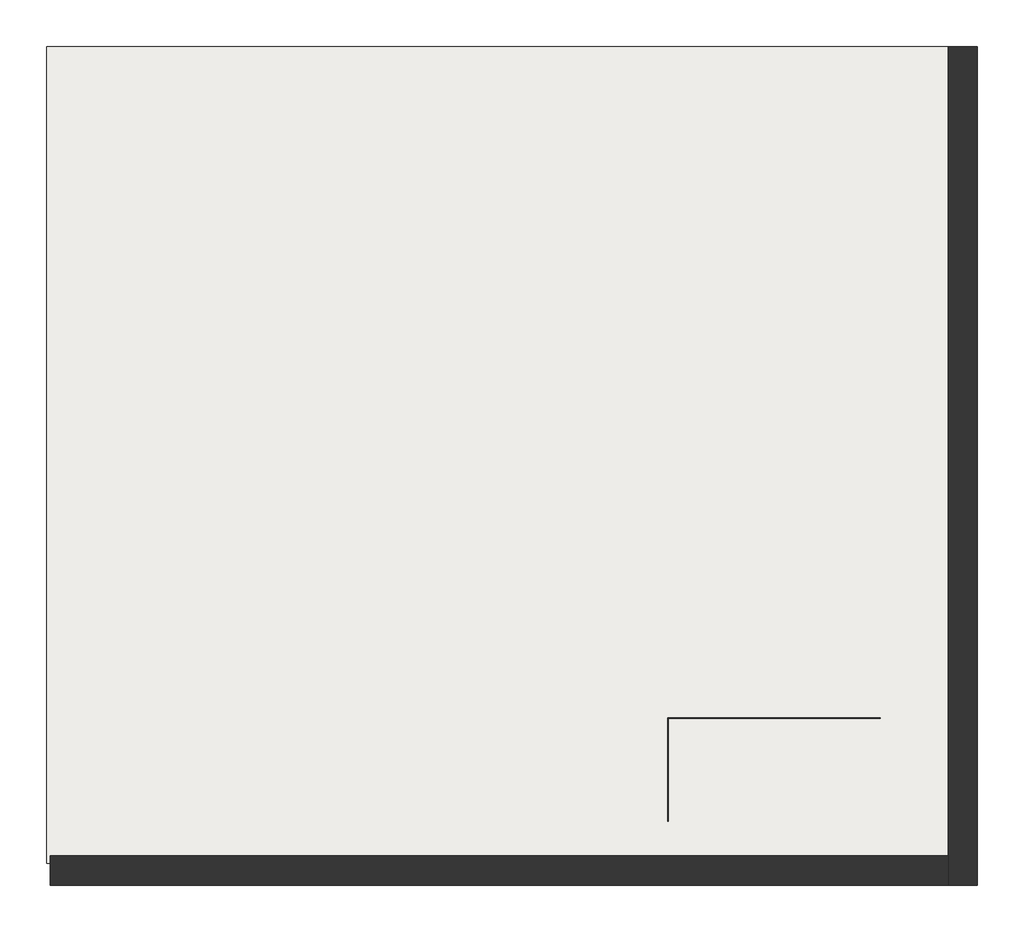
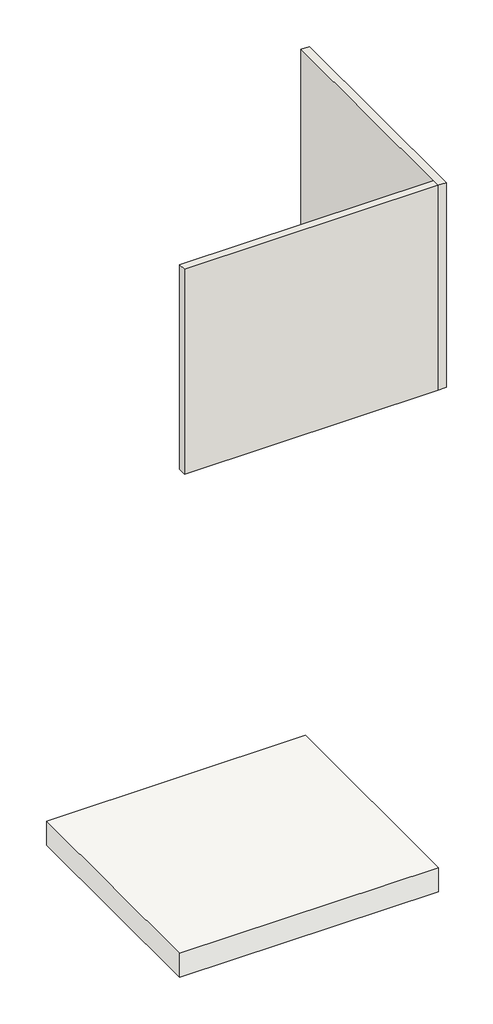
# One storey: 4 walls, 1 slab.
"""IFC4 building model written with IfcOpenShell, lengths in millimetres."""

from ifc_helpers import new_model, si_unit, frame, origin, origin_with_axes, place, context, project, spatial, polyline, outline, extrude, faceted_brep, element, save

model = new_model("IFC4")

# Units and contexts
model_context = context("Model", 3, world=origin())
ifc_project = project(units=[si_unit("LENGTHUNIT", "METRE", prefix="MILLI")], contexts=[model_context])

# Site, building, storey
site = spatial("IfcSite", under=ifc_project)
building = spatial("IfcBuilding", under=site)
storey = spatial("IfcBuildingStorey", under=building, Name="Döşeme", Elevation=0.0)

# Slab
placement = place(None, origin())
element("IfcSlab", 1, ObjectType="Generic - 12\"", at=placement, inside=storey, context=model_context, shape_type="SweptSolid", body=[
    extrude(outline(polyline([(23868.9519544, 5821.7472359), (23868.9519544, 3048.0496219), (20756.9519544, 3048.0496219), (20756.9519544, 5821.7472359), (23868.9519544, 5821.7472359)])), frame((0.0, 0.0, -6432.6532819), z_axis=(0.0, 0.0, 1.0), x_axis=(1.0, 0.0, 0.0)), (0.0, 0.0, 1.0), 304.8),
])

# Walls
element("IfcWall", 2, ObjectType="aa Marble  - 20 mm Siyah", at=placement, inside=storey, context=model_context, shape_type="Brep", body=[
    faceted_brep([(22868.9519544, 3189.0125888, 0.0), (22868.9519544, 3538.0125888, 0.0), (22868.9519544, 3540.0125888, 0.0), (22868.9519544, 3540.0125888, 390.0), (22868.9519544, 3538.0125888, 390.0), (22868.9519544, 3189.0125888, 390.0), (22866.9519544, 3189.0125888, 0.0), (22866.9519544, 3189.0125888, 390.0), (22866.9519544, 3540.0125888, 390.0), (22866.9519544, 3540.0125888, 0.0)], [[[0, 1, 2, 3, 4, 5]], [[6, 7, 8, 9]], [[3, 2, 9, 8]], [[2, 1, 0, 6, 9]], [[5, 4, 3, 8, 7]], [[0, 5, 7, 6]]]),
])
element("IfcWall", 3, ObjectType="aa Marble  - 20 mm Siyah", at=placement, inside=storey, context=model_context, shape_type="SweptSolid", body=[
    extrude(outline(polyline([(23587.9519544, 3538.0125888), (22868.9519544, 3538.0125888), (22868.9519544, 3540.0125888), (23587.9519544, 3540.0125888), (23587.9519544, 3538.0125888)])), origin_with_axes(), (0.0, 0.0, 1.0), 390.0),
])
element("IfcWall", 4, ObjectType="Generic - 100mm", at=placement, inside=storey, context=model_context, shape_type="Brep", body=[
    faceted_brep([(23818.9519544, 5821.7472359, 0.0), (23818.9519544, 3071.7472359, 0.0), (23818.9519544, 2971.7472359, 0.0), (23818.9519544, 2971.7472359, 2600.0), (23818.9519544, 3071.7472359, 2600.0), (23818.9519544, 5821.7472359, 2600.0), (23918.9519544, 5821.7472359, 0.0), (23918.9519544, 5821.7472359, 2600.0), (23918.9519544, 2971.7472359, 2600.0), (23918.9519544, 2971.7472359, 0.0)], [[[0, 1, 2, 3, 4, 5]], [[6, 7, 8, 9]], [[2, 1, 0, 6, 9]], [[5, 4, 3, 8, 7]], [[0, 5, 7, 6]], [[3, 2, 9, 8]]]),
])
element("IfcWall", 5, ObjectType="Generic - 100mm", at=placement, inside=storey, context=model_context, shape_type="SweptSolid", body=[
    extrude(outline(polyline([(20768.9519544, 3071.7472359), (23818.9519544, 3071.7472359), (23818.9519544, 2971.7472359), (20768.9519544, 2971.7472359), (20768.9519544, 3071.7472359)])), origin_with_axes(), (0.0, 0.0, 1.0), 2600.0),
])

save(model, "model.ifc")

# Revit data of these elements
# Project information
#   Organization Name = "Organization Name"
#   Organization Description = "Organization Description"
#   Building Name = "Building Name"
#   Project Issue Date = "Issue Date"
#   Project Status = "Project Status"
#   Client Name = "Client Name"
#   Project Address = "Enter address here\nAddress Line 2"
#   Project Name = "Project Name"
#   Project Number = "Project Number"
# Type "Generic - 12\""
#   Description = "Generic Floor (Material By Category), 12\" thick"
#   Assembly Code = "B1010"
#   Type Mark = "G01"
#   Function = 0
#   Layers, outside or top first: 30.48 cm no material (function 1)
# Type "aa Marble  - 20 mm Siyah"
#   Description = "Generic Wall (Material By Category), 200mm thick"
#   Assembly Code = "B2010"
#   Type Mark = "G06"
#   Layers, outside or top first: 0.2 cm "aa Marble 2 cm Siyah" (function 1)
# Type "Generic - 100mm"
#   Description = "Generic Wall (Material By Category), 100mm thick"
#   Assembly Code = "B2010"
#   Type Mark = "G01"
#   Layers, outside or top first: 10 cm no material (function 1)
# Element 1 (IfcSlab, "Generic - 12\"")
#   Height Offset From Level = -612.7853 cm
#   Phase Created = New Construction
#   Materials on its faces: "Default Floor"
# Element 2 (IfcWall, "aa Marble  - 20 mm Siyah")
#   Top Offset = 0 cm
#   Base Offset = 0 cm
#   wall height = 36 cm
#   Phase Created = New Construction
#   Base Constraint = Döşeme
#   Top Constraint = Küpeşte
#   Materials on its faces: "aa Marble 2 cm Siyah"
# Element 3 (IfcWall, "aa Marble  - 20 mm Siyah")
#   Top Offset = 3 cm
#   Base Offset = 0 cm
#   wall height = 39 cm
#   Phase Created = New Construction
#   Base Constraint = Döşeme
#   Top Constraint = Küpeşte
#   Materials on its faces: "aa Marble 2 cm Siyah"
# Elements 4, 5 (IfcWall, "Generic - 100mm")
#   Top Offset = 0 cm
#   Base Offset = 0 cm
#   Unconnected Height = 260 cm
#   wall height = 260 cm
#   Phase Created = New Construction
#   Base Constraint = Döşeme
#   Materials on its faces: "Default Wall"
# Materials
#   "aa Marble 2 cm Siyah": class "Stone", colour RGB 120 120 120, transparency 0, Description = "Marble, polished veined, stacked", Cost = 0
#   "Default Floor": class "Miscellaneous", colour RGB 128 128 128, transparency 0, Cost = 0
#   "Default Wall": class "Miscellaneous", colour RGB 192 192 192, transparency 0, Cost = 0
